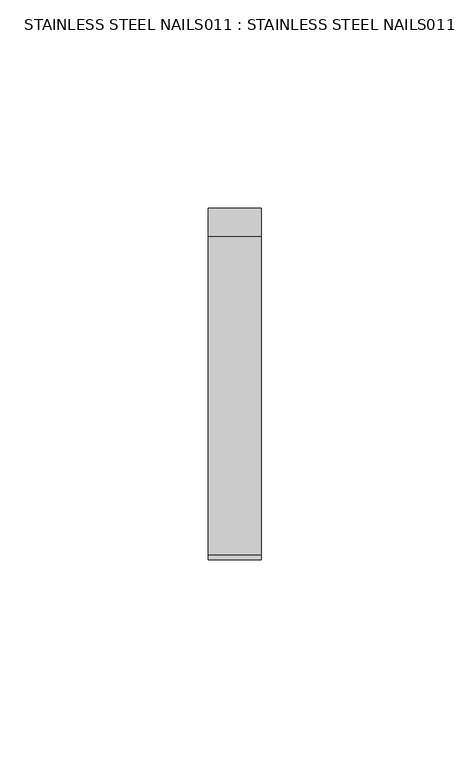
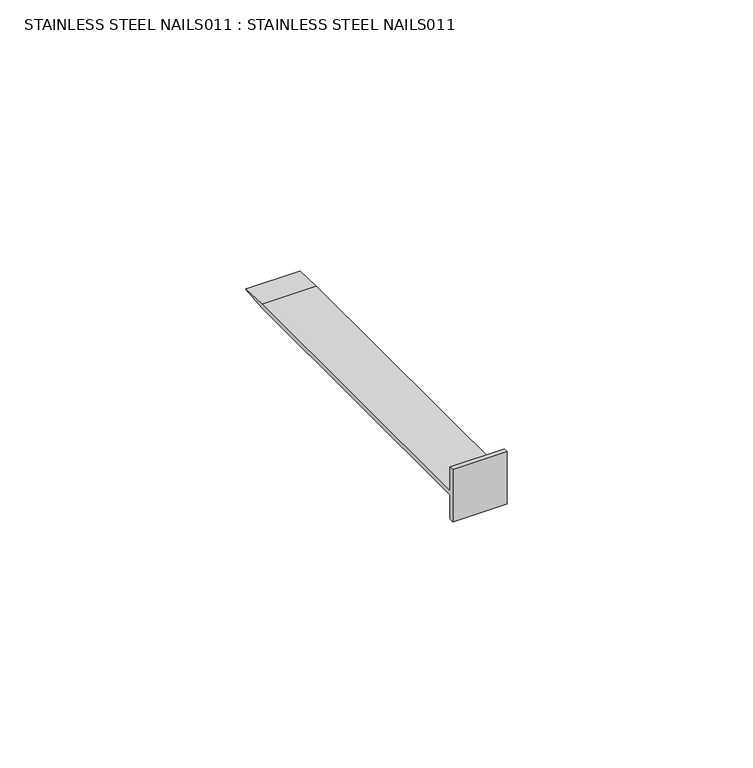
"""IFC4 building model written with IfcOpenShell, lengths in millimetres: proxy geometry, STAINLESS STEEL NAILS011 : STAINLESS STEEL NAILS011."""

from ifc_helpers import new_model, si_unit, frame, origin, place, context, project, spatial, polyline, outline, extrude, source, transform, mapped, element, save


def stainless_steel_nails011_stainless_steel_nails011_743e7744(model_context):
    return source(origin(), model_context, "Body", "SweptSolid", [
        extrude(outline(polyline([(-5577.1765463, 40184.7938624), (-5577.1765463, 40197.7922463), (-5576.0933476, 40197.7922463), (-5576.0933476, 40191.8346536), (-5499.5272732, 40191.8346536), (-5492.898107, 40191.472848), (-5499.5272732, 40190.751455), (-5576.0933476, 40190.751455), (-5576.0933476, 40184.7938624), (-5577.1765463, 40184.7938624)])), frame((14383.0178845, 0.0, 0.0), z_axis=(1.0, 0.0, 0.0), x_axis=(0.0, 1.0, 0.0)), (0.0, 0.0, 1.0), 12.7),
    ])


if __name__ == "__main__":
    model = new_model("IFC4")
    model_context = context("Model", 3, world=origin())
    ifc_project = project(units=[si_unit("LENGTHUNIT", "METRE", prefix="MILLI")], contexts=[model_context])
    site = spatial("IfcSite", under=ifc_project)
    building = spatial("IfcBuilding", under=site)
    placement = place(None, origin())
    stainless_steel_nails011_stainless_steel_nails011_shape = stainless_steel_nails011_stainless_steel_nails011_743e7744(model_context)
    element("IfcBuildingElementProxy", 1, Name="STAINLESS STEEL NAILS011 : STAINLESS STEEL NAILS011", ObjectType="STAINLESS STEEL NAILS011 : STAINLESS STEEL NAILS011", at=placement, inside=building, context=model_context, shape_type="MappedRepresentation", body=[
        mapped(stainless_steel_nails011_stainless_steel_nails011_shape, transform((0.0, 0.0, 0.0), x_axis=(1.0, 0.0, 0.0), y_axis=(0.0, 1.0, 0.0), z_axis=(0.0, 0.0, 1.0))),
    ])
    save(model, "model.ifc")

# Revit data of these elements
# Type "STAINLESS STEEL NAILS011 : STAINLESS STEEL NAILS011"
#   NameOverride = "STAINLESS STEEL NAILS011"
# Element 1 (IfcBuildingElementProxy, "STAINLESS STEEL NAILS011 : STAINLESS STEEL NAILS011")
#   Materials on its faces: "1 3/4\" STAINLESS STEEL RINGSHANK 5D COMMON NAILS @ 4\" (101.6MM) O.C. FIRESTONE PROVIDED MAX., 1/2\" STAGGERED"
# Materials
#   "1 3/4\" STAINLESS STEEL RINGSHANK 5D COMMON NAILS @ 4\" (101.6MM) O.C. FIRESTONE PROVIDED MAX., 1/2\" STAGGERED": class "Unassigned", colour RGB 255 255 255, transparency 0
